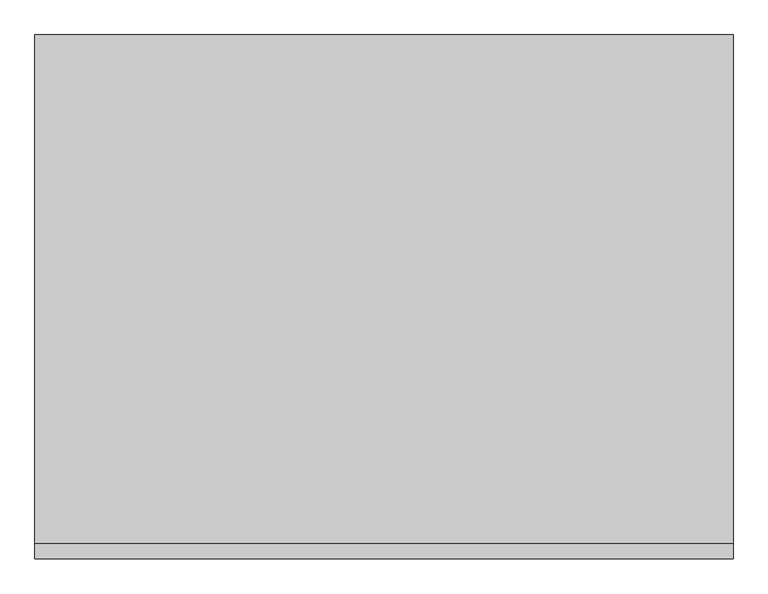
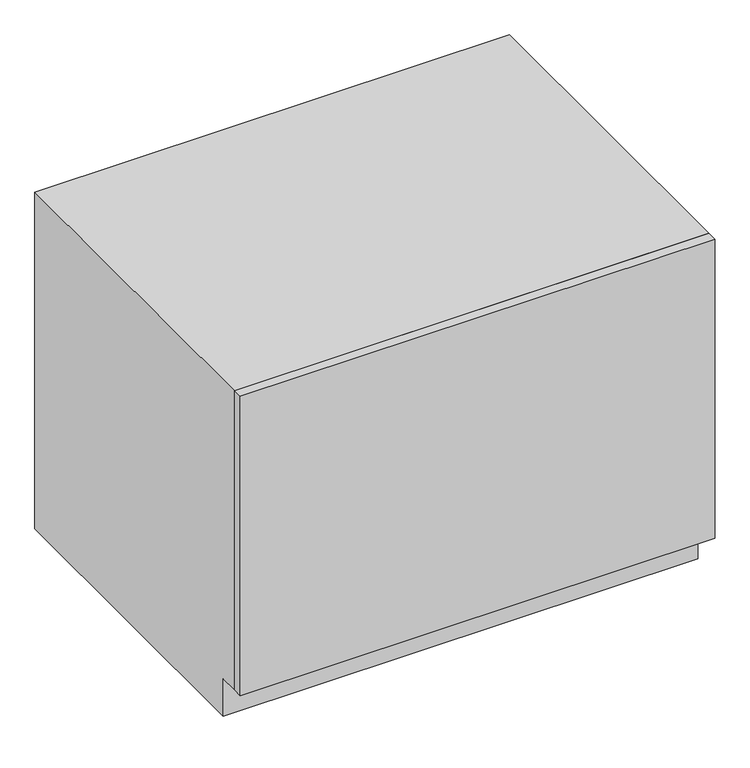
"""IFC4 building model written with IfcOpenShell, lengths in millimetres: furniture geometry, OD_CW_Base Cabinet : OD_CW_Base Cabinet."""

from ifc_helpers import new_model, si_unit, frame, origin, place, context, project, spatial, polyline, outline, extrude, source, transform, mapped, element, save


def furniture_7cfe2ffe(model_context):
    return source(origin(), model_context, "Body", "SweptSolid", [
        extrude(outline(polyline([(18.7377049, -279.4), (1237.9377049, -279.4), (1237.9377049, -304.8), (18.7377049, -304.8), (18.7377049, -279.4)])), frame((0.0, 0.0, 101.6), z_axis=(0.0, 0.0, 1.0), x_axis=(1.0, 0.0, 0.0)), (0.0, 0.0, 1.0), 812.8),
        extrude(outline(polyline([(-279.4, 914.4), (609.6, 914.4), (609.6, 0.0), (-228.6, 0.0), (-228.6, 101.6), (-279.4, 101.6), (-279.4, 914.4)])), frame((18.7377049, 0.0, 0.0), z_axis=(1.0, 0.0, 0.0), x_axis=(0.0, 1.0, 0.0)), (0.0, 0.0, 1.0), 1219.2),
    ])


if __name__ == "__main__":
    model = new_model("IFC4")
    model_context = context("Model", 3, world=origin())
    ifc_project = project(units=[si_unit("LENGTHUNIT", "METRE", prefix="MILLI")], contexts=[model_context])
    site = spatial("IfcSite", under=ifc_project)
    building = spatial("IfcBuilding", under=site)
    placement = place(None, origin())
    furniture_shape = furniture_7cfe2ffe(model_context)
    element("IfcFurniture", 1, ObjectType="OD_CW_Base Cabinet : OD_CW_Base Cabinet", at=placement, inside=building, context=model_context, shape_type="MappedRepresentation", body=[
        mapped(furniture_shape, transform((0.0, 0.0, 0.0), x_axis=(1.0, 0.0, 0.0), y_axis=(0.0, 1.0, 0.0), z_axis=(0.0, 0.0, 1.0))),
    ])
    save(model, "model.ifc")

# Revit data of these elements
# Type "OD_CW_Base Cabinet : OD_CW_Base Cabinet"
#   OD_CW_Width [instance default] = 2' - 10"
#   OD_CW_Length [instance default] = 8' - 0"
#   OD_CW_Height [instance default] = 2' - 3"
#   Depth = 2' - 0"
#   Height = 3' - 0"
#   Width = 4' - 0"
#   OD_CW_Material_Front Panel [instance default] = none
#   OD_CW_Material_Body [instance default] = none
# Element 1 (IfcFurniture, "OD_CW_Base Cabinet : OD_CW_Base Cabinet")
#   OD_CW_Width = 3' - 0"
#   OD_CW_Length = 4' - 0"
#   OD_CW_Height = 3' - 0"
#   OD_CW_Material_Body = SAUTE COOLER
#   Materials on its faces: "SAUTE COOLER", "CASEWORK"
# Materials
#   "SAUTE COOLER": class "Generic", colour RGB 187 187 187, transparency 0, Cost = 0
#   "CASEWORK": class "Generic", colour RGB 181 181 181, transparency 0, Cost = 0
